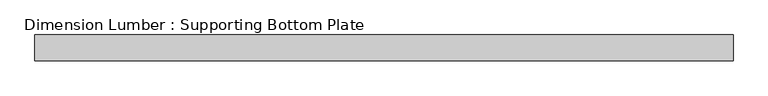
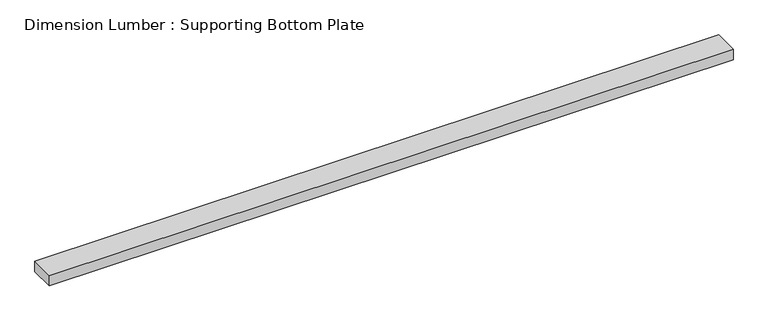
"""IFC4 building model written with IfcOpenShell, lengths in millimetres: beam geometry, Dimension Lumber : Supporting Bottom Plate."""

import ifcopenshell
import ifcopenshell.guid

model = None  # the IFC model being written
_history = None  # IfcOwnerHistory: only IFC2X3 demands one
_inside = {}  # id of a spatial element -> (the spatial element, [elements in it])
_under = {}  # id of a project, library or spatial element -> (it, [spatial elements below it])
_declared = {}  # id of a project -> (the project, [libraries it declares])
_typed = {}  # id of a type object -> (the type object, [elements of that type])
_made_of = {}  # id of a material, layer set ... -> (it, [elements and type objects made of it])


def new_model(schema):
    """Start an empty IFC model of exactly this schema.

    Asked for "IFC4X3", IfcOpenShell would pick the latest addendum, in which some entities
    have other attributes; the version numbers below select the first issue.
    IFC2X3 requires an IfcOwnerHistory on every rooted entity: one is made here for all.
    """
    global model, _history
    if schema == "IFC4X3":
        model = ifcopenshell.file(schema_version=(4, 3, 0, 0))
    else:
        model = ifcopenshell.file(schema=schema)
    _inside.clear()
    _under.clear()
    _declared.clear()
    _typed.clear()
    _made_of.clear()
    _history = None
    if model.schema == "IFC2X3":
        org = make("IfcOrganization", Name="unknown")
        user = make(
            "IfcPersonAndOrganization",
            ThePerson=make("IfcPerson", FamilyName="unknown"),
            TheOrganization=org,
        )
        app = make(
            "IfcApplication",
            ApplicationDeveloper=org,
            Version="unknown",
            ApplicationFullName="unknown",
            ApplicationIdentifier="unknown",
        )
        _history = make(
            "IfcOwnerHistory",
            OwningUser=user,
            OwningApplication=app,
            ChangeAction="ADDED",
            CreationDate=0,
        )
    return model


def make(cls, **values):
    """One entity of the class cls with the attributes given. An attribute that is None is left unset."""
    return model.create_entity(
        cls, **{name: value for name, value in values.items() if value is not None}
    )


def rooted(cls, **values):
    """An entity with a GlobalId (a new one), such as an element, a storey or a relation."""
    return make(cls, GlobalId=ifcopenshell.guid.new(), OwnerHistory=_history, **values)


def si_unit(unit_type, name, prefix=None):
    """IfcSIUnit, for example si_unit("LENGTHUNIT", "METRE", prefix="MILLI")."""
    return make("IfcSIUnit", UnitType=unit_type, Prefix=prefix, Name=name)


def assignment(units):
    """IfcUnitAssignment: the units of a project."""
    return None if units is None else make("IfcUnitAssignment", Units=units)


def point(xyz):
    """IfcCartesianPoint."""
    return None if xyz is None else make("IfcCartesianPoint", Coordinates=xyz)


def direction(xyz):
    """IfcDirection."""
    return None if xyz is None else make("IfcDirection", DirectionRatios=xyz)


def frame(location, z_axis=None, x_axis=None):
    """IfcAxis2Placement3D, a coordinate frame: its origin and axes. An axis left out is left unset."""
    return make(
        "IfcAxis2Placement3D",
        Location=point(location),
        Axis=direction(z_axis),
        RefDirection=direction(x_axis),
    )


def origin():
    """The frame at (0, 0, 0) with its axes left unset."""
    return frame((0.0, 0.0, 0.0))


def place(relative_to, where):
    """IfcLocalPlacement: puts the frame where relative to a parent placement (None: the world)."""
    return make(
        "IfcLocalPlacement", PlacementRelTo=relative_to, RelativePlacement=where
    )


def context(
    kind, dimensions, precision=None, world=None, true_north=None, identifier=None
):
    """IfcGeometricRepresentationContext, for example the 3D "Model" context."""
    return make(
        "IfcGeometricRepresentationContext",
        ContextIdentifier=identifier,
        ContextType=kind,
        CoordinateSpaceDimension=dimensions,
        Precision=precision,
        WorldCoordinateSystem=world,
        TrueNorth=true_north,
    )


def project(units=None, contexts=None):
    """IfcProject with its units and contexts."""
    return rooted(
        "IfcProject",
        Name="project",
        RepresentationContexts=contexts,
        UnitsInContext=assignment(units),
    )


def spatial(cls, under=None, at=None, **own):
    """A site, building, storey or space (cls), placed at a placement, below another one or the project."""
    s = rooted(cls, ObjectPlacement=at, **own)
    if under is not None:
        _under.setdefault(under.id(), (under, []))[1].append(s)
    return s


def polyline(points):
    """IfcPolyline through the points."""
    return make("IfcPolyline", Points=[point(p) for p in points])


def outline(outer, holes=None, kind="AREA"):
    """IfcArbitraryClosedProfileDef: a profile drawn as a closed curve; with holes, ...WithVoids."""
    if holes is None:
        return make("IfcArbitraryClosedProfileDef", ProfileType=kind, OuterCurve=outer)
    return make(
        "IfcArbitraryProfileDefWithVoids",
        ProfileType=kind,
        OuterCurve=outer,
        InnerCurves=holes,
    )


def extrude(swept, where, along, depth):
    """IfcExtrudedAreaSolid: the profile swept, set in the frame where, extruded along a direction by depth."""
    return make(
        "IfcExtrudedAreaSolid",
        SweptArea=swept,
        Position=where,
        ExtrudedDirection=direction(along),
        Depth=depth,
    )


def shape(context_of_items, identifier, shape_type, items):
    """IfcShapeRepresentation: the items that make up one representation, for example the "Body"."""
    return make(
        "IfcShapeRepresentation",
        ContextOfItems=context_of_items,
        RepresentationIdentifier=identifier,
        RepresentationType=shape_type,
        Items=items,
    )


def source(mapping_origin, context_of_items, identifier, shape_type, items):
    """IfcRepresentationMap: a shape defined once, which mapped items show again and again."""
    return make(
        "IfcRepresentationMap",
        MappingOrigin=mapping_origin,
        MappedRepresentation=shape(context_of_items, identifier, shape_type, items),
    )


def transform(
    local_origin,
    x_axis=None,
    y_axis=None,
    z_axis=None,
    scale=None,
    scale2=None,
    scale3=None,
    uniform=True,
):
    """IfcCartesianTransformationOperator3D, or its non-uniform kind. x_axis, y_axis, z_axis: its Axis1, 2, 3."""
    if uniform:
        return make(
            "IfcCartesianTransformationOperator3D",
            Axis1=direction(x_axis),
            Axis2=direction(y_axis),
            LocalOrigin=point(local_origin),
            Scale=scale,
            Axis3=direction(z_axis),
        )
    return make(
        "IfcCartesianTransformationOperator3DnonUniform",
        Axis1=direction(x_axis),
        Axis2=direction(y_axis),
        LocalOrigin=point(local_origin),
        Scale=scale,
        Axis3=direction(z_axis),
        Scale2=scale2,
        Scale3=scale3,
    )


def mapped(mapping_source, mapping_target):
    """IfcMappedItem: shows the shape of a source again, moved by a transform."""
    return make(
        "IfcMappedItem", MappingSource=mapping_source, MappingTarget=mapping_target
    )


def made_of(thing, what):
    """Note that an element or type object is made of a material, layer set ...; save() writes the relation."""
    if what is not None:
        _made_of.setdefault(what.id(), (what, []))[1].append(thing)
    return thing


def element(
    cls,
    number,
    at=None,
    inside=None,
    cuts=None,
    type_object=None,
    material=None,
    context=None,
    identifier="Body",
    shape_type=None,
    held_by="IfcProductDefinitionShape",
    body=None,
    shapes=None,
    **own,
):
    """One element of the class cls, such as IfcWall. Its Tag is "e" and its number.

    at: its placement. inside: the storey or other place that contains it. cuts: it is an
    opening in that element (IfcRelVoidsElement). A single representation is given by context,
    identifier, shape_type and body (its items); several are given by shapes. held_by: the class
    of the entity that holds the representations. save() writes the other relations.
    """
    e = rooted(cls, Tag="e%d" % number, ObjectPlacement=at, **own)
    if body is not None:
        shapes = [shape(context, identifier, shape_type, body)]
    if shapes is not None:
        e.Representation = make(held_by, Representations=shapes)
    if inside is not None:
        _inside.setdefault(inside.id(), (inside, []))[1].append(e)
    if cuts is not None:
        rooted(
            "IfcRelVoidsElement", RelatingBuildingElement=cuts, RelatedOpeningElement=e
        )
    if type_object is not None:
        _typed.setdefault(type_object.id(), (type_object, []))[1].append(e)
    return made_of(e, material)


def aggregate(whole, parts):
    """IfcRelAggregates: a whole, such as a stair, and the parts it consists of."""
    return rooted("IfcRelAggregates", RelatingObject=whole, RelatedObjects=parts)


def save(model, path):
    """Write the relations noted so far, then the file.

    IfcRelAggregates (storeys below a building ...), IfcRelContainedInSpatialStructure (elements
    in a storey), IfcRelDefinesByType, IfcRelAssociatesMaterial and IfcRelDeclares: one each for
    every whole, place, type object, material and project.
    """
    for whole, parts in _under.values():
        aggregate(whole, parts)
    for where, things in _inside.values():
        rooted(
            "IfcRelContainedInSpatialStructure",
            RelatedElements=things,
            RelatingStructure=where,
        )
    for kind, things in _typed.values():
        rooted("IfcRelDefinesByType", RelatedObjects=things, RelatingType=kind)
    for what, things in _made_of.values():
        rooted("IfcRelAssociatesMaterial", RelatedObjects=things, RelatingMaterial=what)
    for by, libraries in _declared.values():
        rooted("IfcRelDeclares", RelatingContext=by, RelatedDefinitions=libraries)
    model.write(path)


def dimension_lumber_supporting_bottom_plate_83ad6fc0(model_context):
    return source(origin(), model_context, "Body", "SweptSolid", [
        extrude(outline(polyline([(1226.5374575, -44.45), (-1182.0874575, -44.45), (-1182.0874575, 44.45), (1226.5374575, 44.45), (1226.5374575, -44.45)])), frame((0.0, 0.0, -19.05), z_axis=(0.0, 0.0, 1.0), x_axis=(1.0, 0.0, 0.0)), (0.0, 0.0, 1.0), 38.1),
    ])


if __name__ == "__main__":
    model = new_model("IFC4")
    model_context = context("Model", 3, world=origin())
    ifc_project = project(units=[si_unit("LENGTHUNIT", "METRE", prefix="MILLI")], contexts=[model_context])
    site = spatial("IfcSite", under=ifc_project)
    building = spatial("IfcBuilding", under=site)
    placement = place(None, origin())
    dimension_lumber_supporting_bottom_plate_shape = dimension_lumber_supporting_bottom_plate_83ad6fc0(model_context)
    element("IfcBeam", 1, ObjectType="Dimension Lumber : Supporting Bottom Plate", at=placement, inside=building, context=model_context, shape_type="MappedRepresentation", body=[
        mapped(dimension_lumber_supporting_bottom_plate_shape, transform((0.0, 0.0, 0.0), x_axis=(1.0, 0.0, 0.0), y_axis=(0.0, 1.0, 0.0), z_axis=(0.0, 0.0, 1.0))),
    ])
    save(model, "model.ifc")

# Revit data of these elements
# Type "Dimension Lumber : Supporting Bottom Plate"
#   Assembly Code = "B10"
#   A = 0.0364583 SF
#   Length [instance default] = 5' - 0"
#   b = 0' - 3 1/2"
#   d = 0' - 1 1/2"
#   Structural Material [instance default] = Softwood, Lumber
# Element 1 (IfcBeam, "Dimension Lumber : Supporting Bottom Plate")
#   Structural Material = Douglas Fir #2
#   Materials on its faces: "Douglas Fir #2"
# Materials
#   "Softwood, Lumber": class "Wood", colour RGB 223 192 134, transparency 0, Description = "Pinus Echinata", Cost = 0
#   "Douglas Fir #2": class "Wood", colour RGB 223 192 134, transparency 0, Description = "Pinus Echinata", Cost = 0
